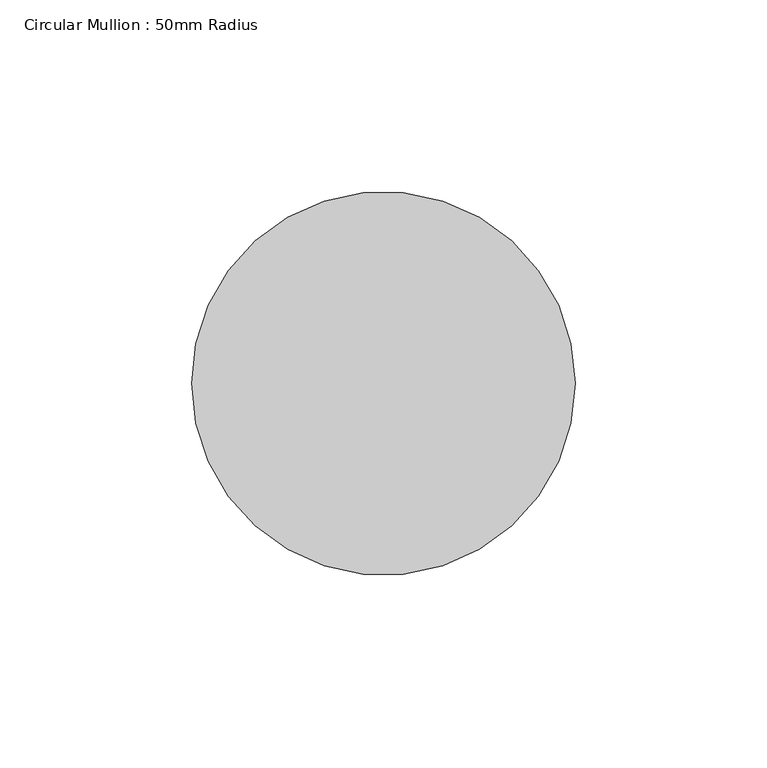
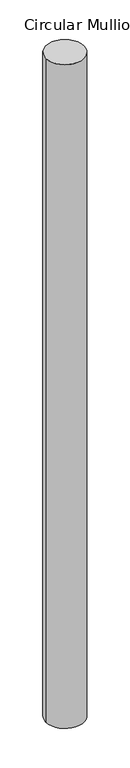
"""IFC4 building model written with IfcOpenShell, lengths in millimetres: member geometry, Circular Mullion : 50mm Radius."""

from ifc_helpers import new_model, si_unit, point, frame, origin, origin_2d, place, context, project, spatial, circle_curve, trimmed, segment, composite_curve, outline, extrude, source, transform, mapped, element, save


def circular_mullion_50mm_radius_5fb068b1(model_context):
    return source(origin(), model_context, "Body", "SweptSolid", [
        extrude(outline(composite_curve([segment(trimmed(circle_curve(origin_2d(), 50.0), [point((50.0, 0.0))], [point((-50.0, 0.0))], False, "CARTESIAN"), True, "CONTINUOUS"), segment(trimmed(circle_curve(origin_2d(), 50.0), [point((-50.0, 0.0))], [point((50.0, 0.0))], False, "CARTESIAN"), True, "CONTINUOUS")], self_intersect=False)), frame((0.0, 0.0, -1847.4795039), z_axis=(0.0, 0.0, 1.0), x_axis=(1.0, 0.0, 0.0)), (0.0, 0.0, 1.0), 1847.4795039),
    ])


if __name__ == "__main__":
    model = new_model("IFC4")
    model_context = context("Model", 3, world=origin())
    ifc_project = project(units=[si_unit("LENGTHUNIT", "METRE", prefix="MILLI")], contexts=[model_context])
    site = spatial("IfcSite", under=ifc_project)
    building = spatial("IfcBuilding", under=site)
    placement = place(None, origin())
    circular_mullion_50mm_radius_shape = circular_mullion_50mm_radius_5fb068b1(model_context)
    element("IfcMember", 1, ObjectType="Circular Mullion : 50mm Radius", at=placement, inside=building, context=model_context, shape_type="MappedRepresentation", body=[
        mapped(circular_mullion_50mm_radius_shape, transform((0.0, 0.0, 0.0), x_axis=(1.0, 0.0, 0.0), y_axis=(0.0, 1.0, 0.0), z_axis=(0.0, 0.0, 1.0))),
    ])
    save(model, "model.ifc")

# Revit data of these elements
# Type "Circular Mullion : 50mm Radius"
#   built-in parameter 1007350 = 0.164042 (stored number, unit not read)
# Element 1 (IfcMember, "Circular Mullion : 50mm Radius")
#   Materials on its faces: "Aluminium"
# Materials
#   "Aluminium": class "Metal", colour RGB 247 247 247, transparency 0, Description = "Aluminium 6061", Cost = 0
